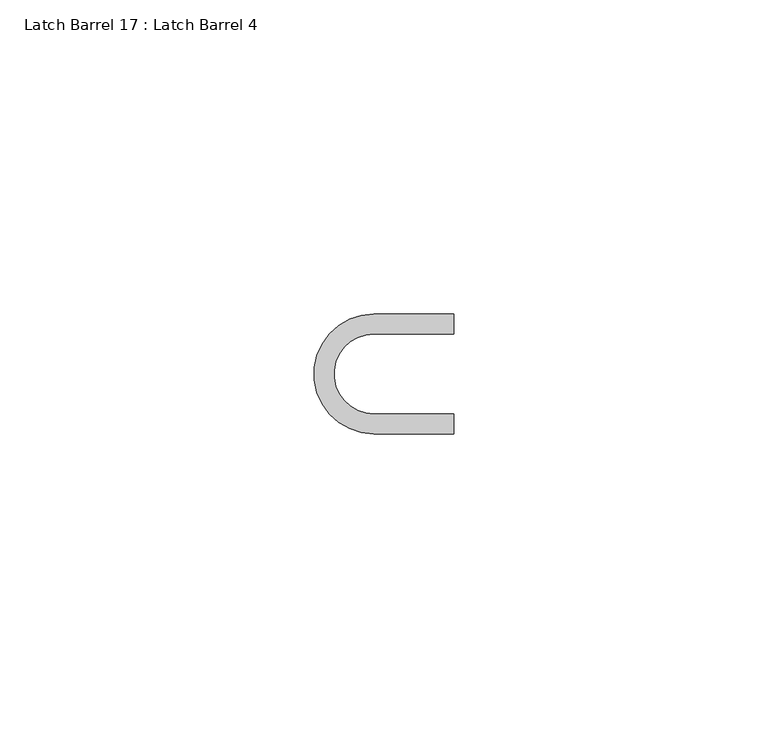
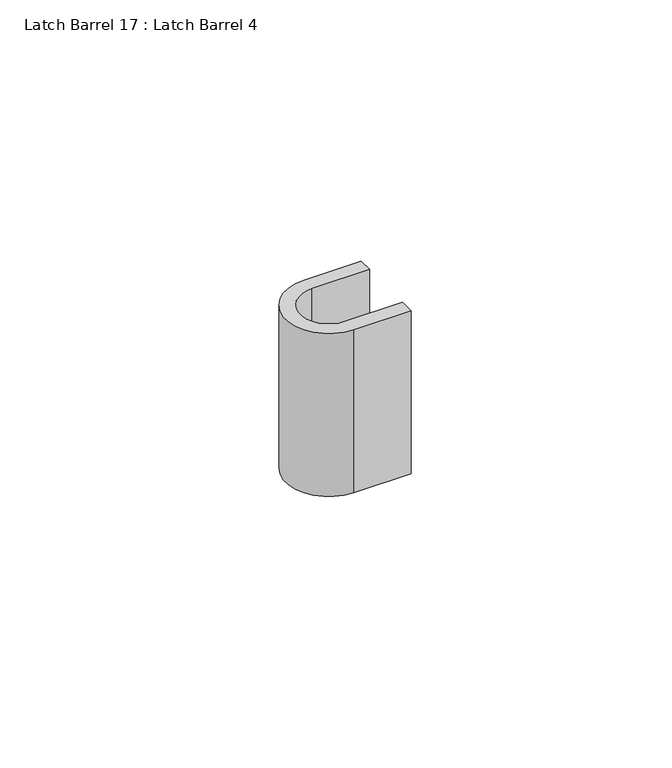
"""IFC4 building model written with IfcOpenShell, lengths in millimetres: proxy geometry, Latch Barrel 17 : Latch Barrel 4."""

from ifc_helpers import new_model, si_unit, point, frame, frame_2d, origin, place, context, project, spatial, polyline, circle_curve, trimmed, segment, composite_curve, outline, extrude, source, transform, mapped, element, save


def latch_barrel_17_latch_barrel_4_aacd6dec(model_context):
    return source(origin(), model_context, "Body", "SweptSolid", [
        extrude(outline(composite_curve([segment(trimmed(circle_curve(frame_2d((587309.5435739, -535163.4663841)), 6.35), [point((587309.5435739, -535157.1163841))], [point((587309.5435739, -535169.8163841))], True, "CARTESIAN"), True, "CONTINUOUS"), segment(polyline([(587309.5435739, -535169.8163841), (587322.2435739, -535169.8163841), (587322.2435739, -535172.9913841), (587309.5435739, -535172.9913841)]), True, "CONTINUOUS"), segment(trimmed(circle_curve(frame_2d((587309.5435739, -535163.4663841)), 9.525), [point((587309.5435739, -535172.9913841))], [point((587309.5435739, -535153.9413841))], False, "CARTESIAN"), True, "CONTINUOUS"), segment(polyline([(587309.5435739, -535153.9413841), (587322.2435739, -535153.9413841), (587322.2435739, -535157.1163841), (587309.5435739, -535157.1163841)]), True, "CONTINUOUS")], self_intersect=False)), frame((0.0, 0.0, 241.3), z_axis=(0.0, 0.0, 1.0), x_axis=(1.0, 0.0, 0.0)), (0.0, 0.0, 1.0), 38.1),
    ])


if __name__ == "__main__":
    model = new_model("IFC4")
    model_context = context("Model", 3, world=origin())
    ifc_project = project(units=[si_unit("LENGTHUNIT", "METRE", prefix="MILLI")], contexts=[model_context])
    site = spatial("IfcSite", under=ifc_project)
    building = spatial("IfcBuilding", under=site)
    placement = place(None, origin())
    latch_barrel_17_latch_barrel_4_shape = latch_barrel_17_latch_barrel_4_aacd6dec(model_context)
    element("IfcBuildingElementProxy", 1, Name="Latch Barrel 17 : Latch Barrel 4", ObjectType="Latch Barrel 17 : Latch Barrel 4", at=placement, inside=building, context=model_context, shape_type="MappedRepresentation", body=[
        mapped(latch_barrel_17_latch_barrel_4_shape, transform((0.0, 0.0, 0.0), x_axis=(1.0, 0.0, 0.0), y_axis=(0.0, 1.0, 0.0), z_axis=(0.0, 0.0, 1.0))),
    ])
    save(model, "model.ifc")

# Revit data of these elements
# Element 1 (IfcBuildingElementProxy, "Latch Barrel 17 : Latch Barrel 4")
#   Materials on its faces: "GALV. SLIDE BOLT"
# Materials
#   "GALV. SLIDE BOLT": class "Metal", colour RGB 189 187 185, transparency 0, Description = "Carbon steel", Cost = 0
